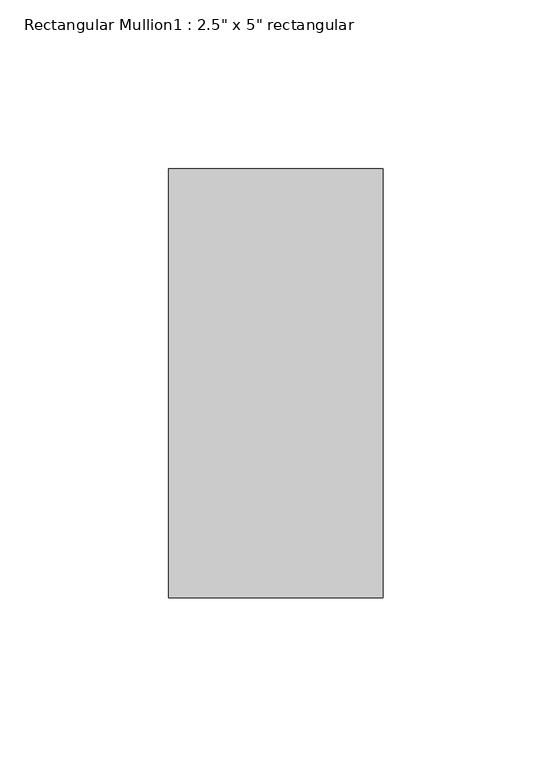
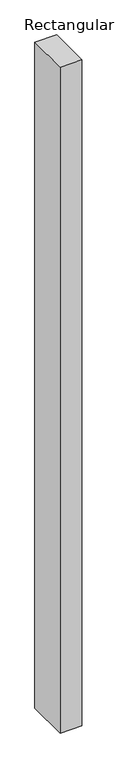
"""IFC4 building model written with IfcOpenShell, lengths in millimetres: member geometry."""

from ifc_helpers import new_model, si_unit, frame, origin, place, context, project, spatial, polyline, outline, extrude, source, transform, mapped, element, save


def member_0efe1817(model_context):
    return source(origin(), model_context, "Body", "SweptSolid", [
        extrude(outline(polyline([(31.75, 63.5), (31.75, -63.5), (-31.75, -63.5), (-31.75, 63.5), (31.75, 63.5)])), frame((0.0, 0.0, -2053.1666667), z_axis=(0.0, 0.0, 1.0), x_axis=(1.0, 0.0, 0.0)), (0.0, 0.0, 1.0), 2053.1666667),
    ])


if __name__ == "__main__":
    model = new_model("IFC4")
    model_context = context("Model", 3, world=origin())
    ifc_project = project(units=[si_unit("LENGTHUNIT", "METRE", prefix="MILLI")], contexts=[model_context])
    site = spatial("IfcSite", under=ifc_project)
    building = spatial("IfcBuilding", under=site)
    placement = place(None, origin())
    member_shape = member_0efe1817(model_context)
    element("IfcMember", 1, ObjectType="Rectangular Mullion1 : 2.5\" x 5\" rectangular", at=placement, inside=building, context=model_context, shape_type="MappedRepresentation", body=[
        mapped(member_shape, transform((0.0, 0.0, 0.0), x_axis=(1.0, 0.0, 0.0), y_axis=(0.0, 1.0, 0.0), z_axis=(0.0, 0.0, 1.0))),
    ])
    save(model, "model.ifc")

# Revit data of these elements
# Type "Rectangular Mullion1 : 2.5\" x 5\" rectangular"
#   built-in parameter 1007304 = 0.416667 (stored number, unit not read)
#   built-in parameter 1007301 = 0.104167 (stored number, unit not read)
#   built-in parameter 1007300 = 0.104167 (stored number, unit not read)
# Element 1 (IfcMember, "Rectangular Mullion1 : 2.5\" x 5\" rectangular")
#   Materials on its faces: "support-frame"
# Materials
#   "support-frame": class "Unassigned", colour RGB 233 233 233, transparency 0, Cost = 0
